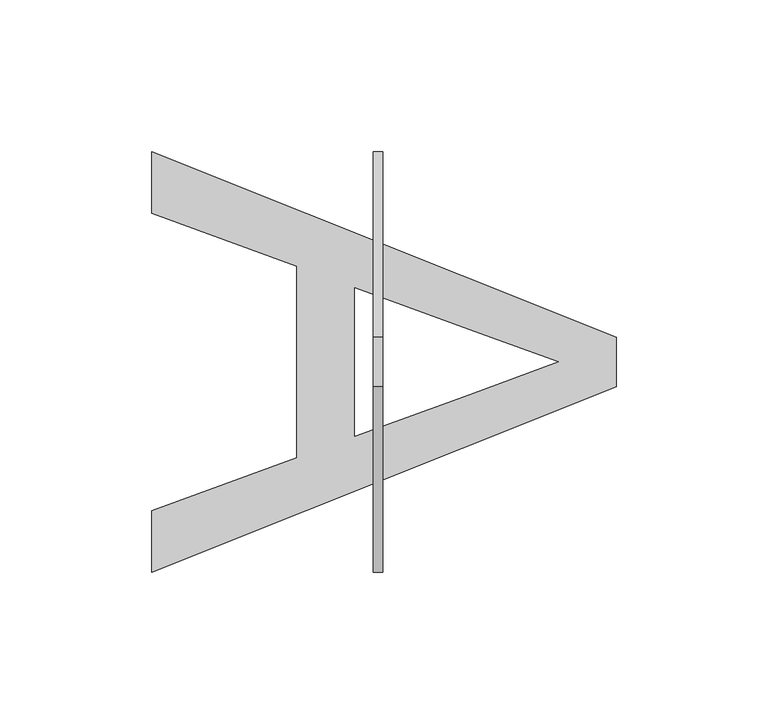
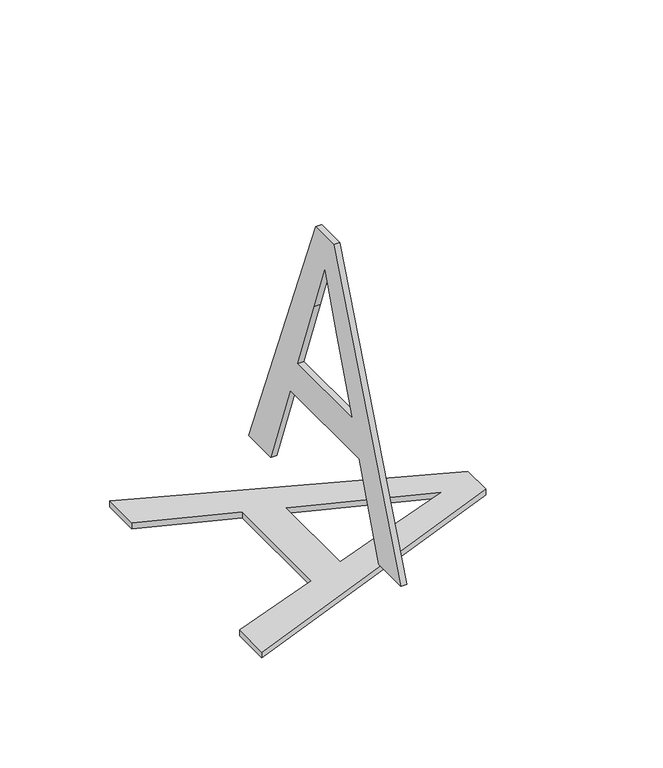
"""IFC4 building model written with IfcOpenShell, lengths in millimetres: proxy geometry, Grid Number2_FedEx : Grid Number2_FedEx."""

from ifc_helpers import new_model, si_unit, frame, origin, origin_with_axes, place, context, project, spatial, polyline, outline, extrude, source, transform, mapped, element, save


def entourage_bd32e15a(model_context):
    return source(origin(), model_context, "Body", "SweptSolid", [
        extrude(outline(polyline([(-184.2739267, 294.1720227), (-31.1785101, 233.0609371), (-31.1785101, 216.7646477), (-184.2739267, 155.6535622), (-184.2739267, 175.8744168), (-136.431609, 193.404141), (-136.431609, 256.4588206), (-184.2739267, 273.9511681), (-184.2739267, 294.1720227)]), holes=[polyline([(-117.2946819, 249.4319802), (-117.2946819, 200.3936046), (-79.6562336, 214.1856477), (-50.3154372, 224.9127924), (-76.3670742, 234.4438791), (-117.2946819, 249.4319802)])]), origin_with_axes(), (0.0, 0.0, 1.0), 3.175),
        extrude(outline(polyline([(294.1720227, 14.2382753), (273.9511681, 14.2382753), (256.4588206, 62.080593), (193.404141, 62.080593), (175.8744168, 14.2382753), (155.6535622, 14.2382753), (216.7646477, 167.333692), (233.0609371, 167.333692), (294.1720227, 14.2382753)]), holes=[polyline([(249.4319802, 81.2175201), (234.4438791, 122.1451278), (224.9127924, 148.1967649), (214.1856477, 118.8559685), (200.3936046, 81.2175201), (249.4319802, 81.2175201)])]), frame((-111.2489267, 0.0, 0.0), z_axis=(1.0, 0.0, 0.0), x_axis=(0.0, 1.0, 0.0)), (0.0, 0.0, 1.0), 3.175),
    ])


if __name__ == "__main__":
    model = new_model("IFC4")
    model_context = context("Model", 3, world=origin())
    ifc_project = project(units=[si_unit("LENGTHUNIT", "METRE", prefix="MILLI")], contexts=[model_context])
    site = spatial("IfcSite", under=ifc_project)
    building = spatial("IfcBuilding", under=site)
    placement = place(None, origin())
    entourage_shape = entourage_bd32e15a(model_context)
    element("IfcBuildingElementProxy", 1, Name="Grid Number2_FedEx : Grid Number2_FedEx", ObjectType="Grid Number2_FedEx : Grid Number2_FedEx", at=placement, inside=building, context=model_context, shape_type="MappedRepresentation", body=[
        mapped(entourage_shape, transform((0.0, 0.0, 0.0), x_axis=(1.0, 0.0, 0.0), y_axis=(0.0, 1.0, 0.0), z_axis=(0.0, 0.0, 1.0))),
    ])
    save(model, "model.ifc")

# Revit data of these elements
# Type "Grid Number2_FedEx : Grid Number2_FedEx"
#   Grid [instance default] = "S"
#   Label Width [instance default] = 1' - 0"
#   Half Box Width2 [instance default] = 0' - 6.13846"
#   Half Box Width [instance default] = 0' - 6"
#   Robust [instance default] = yes
#   Height = 0
#   Assembly Code = ""
# Element 1 (IfcBuildingElementProxy, "Grid Number2_FedEx : Grid Number2_FedEx")
#   Grid = "A"
#   Robust = no
#   Materials on its faces: "Letter"
# Materials
#   "Letter": class "Unassigned", colour RGB 178 187 30, transparency 0, Comments = "Rendering appearance not upgraded "
